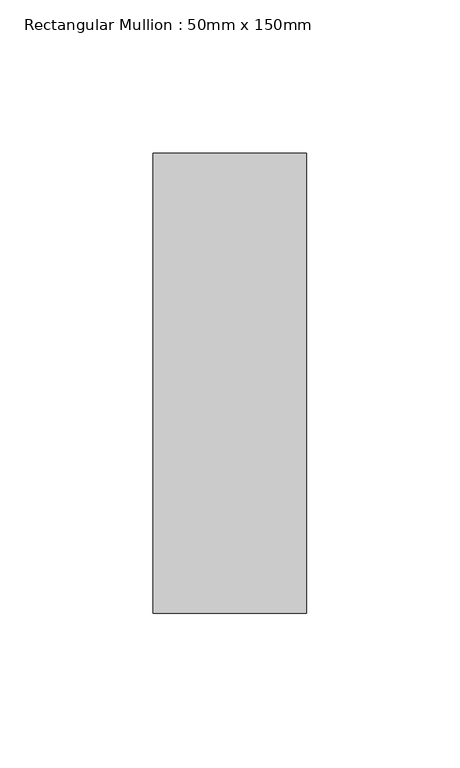
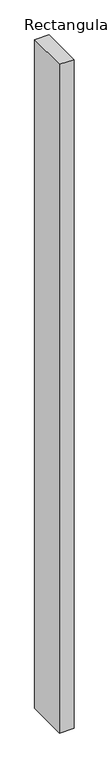
"""IFC4 building model written with IfcOpenShell, lengths in millimetres: member geometry, Rectangular Mullion : 50mm x 150mm."""

from ifc_helpers import new_model, si_unit, frame, origin, place, context, project, spatial, polyline, outline, extrude, source, transform, mapped, element, save


def rectangular_mullion_50mm_x_150mm_448ffc4f(model_context):
    return source(origin(), model_context, "Body", "SweptSolid", [
        extrude(outline(polyline([(0.0, 75.0), (0.0, -75.0), (-50.0, -75.0), (-50.0, 75.0), (0.0, 75.0)])), frame((0.0, 0.0, -2460.0), z_axis=(0.0, 0.0, 1.0), x_axis=(1.0, 0.0, 0.0)), (0.0, 0.0, 1.0), 2460.0),
    ])


if __name__ == "__main__":
    model = new_model("IFC4")
    model_context = context("Model", 3, world=origin())
    ifc_project = project(units=[si_unit("LENGTHUNIT", "METRE", prefix="MILLI")], contexts=[model_context])
    site = spatial("IfcSite", under=ifc_project)
    building = spatial("IfcBuilding", under=site)
    placement = place(None, origin())
    rectangular_mullion_50mm_x_150mm_shape = rectangular_mullion_50mm_x_150mm_448ffc4f(model_context)
    element("IfcMember", 1, ObjectType="Rectangular Mullion : 50mm x 150mm", at=placement, inside=building, context=model_context, shape_type="MappedRepresentation", body=[
        mapped(rectangular_mullion_50mm_x_150mm_shape, transform((0.0, 0.0, 0.0), x_axis=(1.0, 0.0, 0.0), y_axis=(0.0, 1.0, 0.0), z_axis=(0.0, 0.0, 1.0))),
    ])
    save(model, "model.ifc")

# Revit data of these elements
# Type "Rectangular Mullion : 50mm x 150mm"
#   built-in parameter 1007304 = 0.492126 (stored number, unit not read)
#   built-in parameter 1007301 = 0.082021 (stored number, unit not read)
#   built-in parameter 1007300 = 0.082021 (stored number, unit not read)
# Element 1 (IfcMember, "Rectangular Mullion : 50mm x 150mm")
#   Materials on its faces: "Aluminum"
# Materials
#   "Aluminum": class "Metal", colour RGB 244 244 244, transparency 0, Description = "Aluminum 6061", Cost = 0
